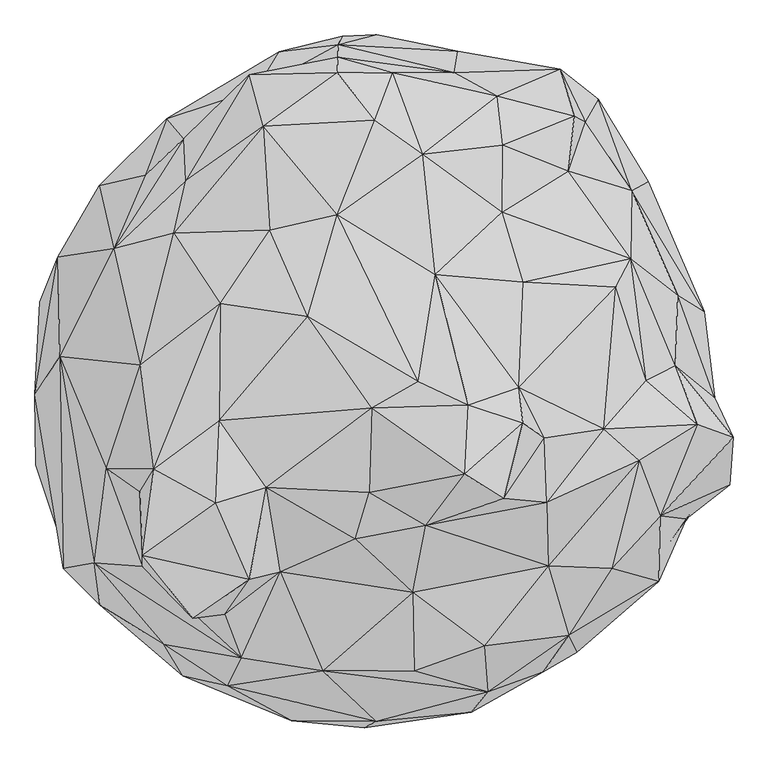
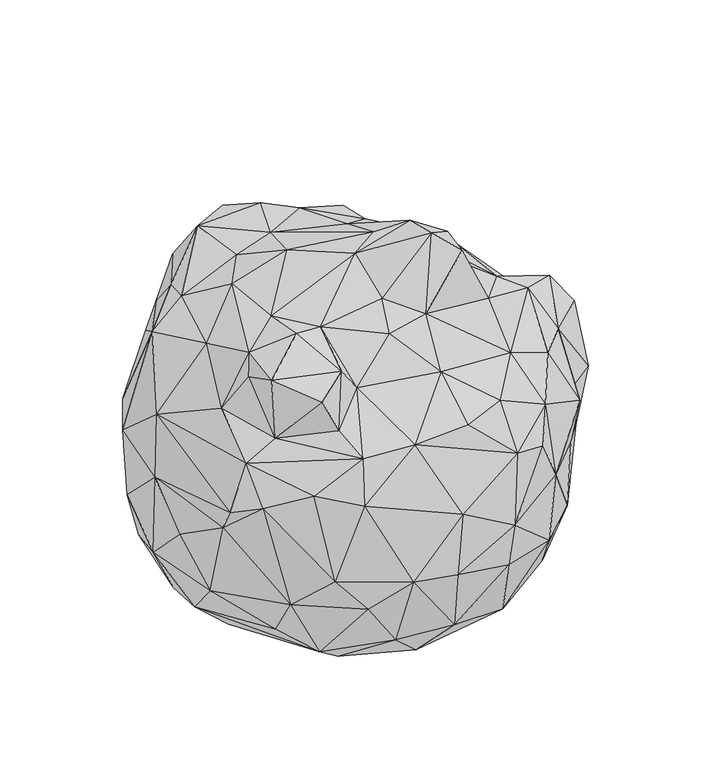
"""IFC4 building model written with IfcOpenShell, lengths in millimetres: geographic element geometry, Enscape AssetDefinition - Bush 001 Balm Bush : Enscape AssetDefinition - Bush 001 Balm Bush."""

from ifc_helpers import new_model, si_unit, origin, place, context, project, spatial, faceted_brep, source, transform, mapped, element, save


def geographic_element_0c4992a3(model_context):
    return source(origin(), model_context, "Body", "Brep", [
        faceted_brep([(-103.2708213, -28.0293748, 87.4930173), (344.7891772, -278.2743871, 87.4930173), (121.6873899, -550.0509143, 87.4930173), (312.7504289, -485.3526056, 87.4930173), (537.6026034, -111.360997, 122.5993857), (31.9034122, 85.9397277, 106.1995625), (483.1260741, 50.9389266, 117.1098575), (301.1055291, 161.4273489, 145.9610015), (-443.3142543, -218.7629938, 87.4930173), (-317.2000349, 6.4054755, 115.6498641), (-249.1122484, 226.8746197, 170.0659692), (94.6265161, 492.8733408, 281.8422019), (390.8439279, 296.7088819, 194.9024647), (518.7944174, 159.3808234, 184.8918945), (213.8534337, 460.0220025, 271.2863088), (425.7422388, 371.6726303, 251.8079579), (571.9012618, 134.5211118, 239.2979264), (542.7101851, 313.1485879, 468.670696), (379.9126446, 478.785485, 348.4884501), (445.0309277, 472.5328982, 451.1599839), (204.6146989, 556.6639304, 384.8151863), (510.0300908, 295.0474024, 639.8970485), (420.6644893, 429.313153, 672.0098257), (371.8031645, 530.8707952, 587.9698992), (650.9532332, 60.9223247, 488.0606234), (599.1232991, 92.9313004, 678.4057021), (508.5837245, 163.8322026, 850.7678509), (387.6252174, 333.4215879, 830.0852776), (398.8237381, 439.2881989, 790.2318835), (258.9309216, 253.3104122, 980.7052612), (260.5757713, 383.2080066, 949.7843385), (249.8932481, 478.099972, 884.2920661), (105.5608988, 366.3907349, 1005.6074858), (299.9075055, 118.1322485, 1021.5417147), (129.529193, 131.8538785, 1082.4985504), (47.3745875, 524.1814256, 883.228898), (12.6913656, 432.1153164, 1015.0117874), (-60.5219491, 248.3438998, 1047.7212667), (165.8966839, 524.0991116, 726.0334492), (-60.8999804, 523.4262943, 976.347208), (-59.549503, 553.7672043, 822.6758242), (-203.7955672, 420.4857647, 1017.4963474), (-230.6382805, 519.813776, 867.0647144), (-58.2677908, 578.6400437, 560.2571964), (-217.2929198, 491.6258454, 723.5295773), (173.101142, 566.0328269, 493.6592281), (15.6866908, 597.2068906, 333.124131), (-172.4721193, 564.8728609, 497.937113), (-50.7058874, 595.2501297, 355.7927608), (-390.5587792, 435.1478517, 548.4309793), (-357.5637639, 396.4434266, 820.2494979), (-343.9708948, 442.8346157, 317.6766038), (-372.1790016, 377.2239387, 247.8975356), (-237.534374, 397.4771798, 235.202238), (-479.7798395, 40.6567864, 115.3686419), (-473.3586311, 183.7875992, 165.3854996), (-502.1672845, 310.5277717, 338.2746279), (-566.3319826, 135.0266039, 225.5846113), (-637.4351978, 79.2079121, 425.8950949), (-601.8330455, 166.0981923, 590.0059342), (-521.4918852, 305.3177297, 587.0153904), (-540.3149724, -20.7758527, 124.5407835), (-645.5538869, -87.3326957, 326.2942135), (-485.3806496, -245.1593429, 111.8686944), (-579.3501139, -210.9759301, 185.881868), (-644.705832, -236.6477698, 479.1609049), (-646.4878321, -100.2570987, 598.8438129), (-594.2829251, -327.2557259, 317.9192841), (-464.2079473, -479.5174897, 227.9132307), (-352.8320491, -542.8832173, 148.7132013), (-455.3643167, -551.6501665, 355.2601039), (-271.4672089, -680.8964014, 353.6209464), (-170.5118865, -666.5790081, 202.0171285), (-285.6132984, -532.9383612, 102.6492417), (-591.2223458, -396.5682685, 580.4986358), (-521.1909413, -507.8048706, 690.6690598), (-591.9779539, -437.338084, 658.8361859), (-359.9068522, -645.4859972, 459.941864), (-148.5068798, -733.5099578, 437.9141033), (-396.7211545, -585.1808786, 738.4177446), (-273.3705044, -665.6394005, 709.523201), (-531.3819647, -427.161932, 807.2852492), (-598.5030532, -26.1186399, 759.1011524), (-508.1710815, -243.2810217, 880.5730343), (-438.2089078, -433.5936904, 865.5333519), (-246.6039956, -610.5666757, 833.7258697), (-88.9153406, -636.6765499, 844.8604345), (-170.9100604, -443.9971745, 956.7247629), (-278.5761952, -526.8044472, 893.348515), (15.429561, -733.9650393, 620.2399731), (231.3562334, -676.6399145, 726.3646126), (86.1066207, -484.4261408, 947.5157857), (88.954322, -636.2065077, 852.5073528), (224.4531512, -587.3548985, 861.1423969), (348.3548462, -432.8074157, 891.8932676), (111.0403612, -353.9148867, 1065.9604073), (-25.0923093, -380.2599907, 1058.245182), (387.8862858, -567.8147078, 777.7100205), (345.3665376, -310.0345433, 1011.2187862), (524.972558, -228.3504009, 935.6176853), (471.6629982, -437.2110367, 852.3084521), (339.2041624, -637.9516721, 691.8114424), (403.8853049, -599.8657942, 542.9646969), (562.8346205, -462.8386199, 667.9671407), (565.5180812, -335.6069624, 842.4683213), (543.7597036, -445.9197521, 519.1505551), (616.3422465, -341.9879079, 634.5546842), (636.9858384, -158.2563668, 898.1446028), (700.1382709, -275.8756578, 628.4427047), (706.8634629, -183.504194, 800.0890613), (632.6106191, -320.7831979, 469.7009921), (496.0250258, -506.0352087, 345.8895385), (597.0824957, -272.9684114, 188.5565519), (694.5405006, -162.4348462, 503.6548376), (666.3972139, -232.2055995, 314.5858049), (671.0886359, -106.4899862, 513.7941837), (594.8883295, -44.487454, 771.445632), (646.2192535, -58.1617877, 356.3556671), (511.9303465, -329.6220005, 145.768255), (406.0667455, -518.4435844, 190.7577068), (220.6544578, -612.2706532, 142.0440227), (380.6358278, -603.4296751, 321.4735389), (184.3929738, -707.8516483, 366.9776917), (11.4893802, -691.2187934, 205.8644295), (-75.4184127, -621.0311055, 106.2972471), (-157.6553881, -553.2301664, 87.4930173), (-7.666158, -746.5350628, 423.5813916), (199.0914494, -717.0593143, 507.3672533), (538.1067991, -72.7551207, 873.780787), (479.3207943, 108.591713, 904.4874907), (455.8838308, -167.5695628, 964.8863077), (291.7309999, -86.5770802, 1084.6892595), (340.4398561, -184.2843294, 1059.3217611), (193.4082955, -120.8397746, 1224.5627642), (298.9223301, -155.5948406, 1171.4243889), (261.9477212, -301.9075692, 1205.515027), (186.9322956, -254.3039024, 1264.8140192), (96.8473852, -75.4188523, 1191.7635202), (6.1829505, -126.3385117, 1176.9108772), (-117.9513335, 51.0777831, 1126.2102127), (-197.9201138, -280.4838419, 1082.4097395), (1.5169365, -289.9889052, 1118.8482046), (-289.5162702, -150.8416384, 1075.7974386), (-296.0483432, -310.9500408, 1113.3135557), (-231.2011719, -458.6890638, 1046.2844372), (-287.4570489, 75.9326741, 1049.9675274), (-416.0194695, -244.8229343, 1048.0645895), (-438.0349815, -411.9614661, 1058.3431721), (-340.1862383, -534.9345207, 1020.7331181), (-443.3633387, -289.6481156, 998.6404777), (-442.3177242, -43.1812182, 965.6659961), (-493.9005673, 182.8322262, 887.7061009), (-377.6369989, 212.3513818, 956.7554593), (-432.6637387, 325.3379762, 786.0648036), (-353.9012969, 314.6484196, 926.5795946), (-191.2693381, 219.0464139, 1032.8195095)], [[[0, 1, 2]], [[3, 1, 4]], [[5, 1, 0]], [[3, 2, 1]], [[1, 6, 4]], [[7, 6, 1]], [[1, 5, 7]], [[8, 9, 0]], [[8, 0, 2]], [[5, 0, 9]], [[10, 7, 5]], [[9, 10, 5]], [[10, 11, 7]], [[12, 7, 11]], [[12, 6, 7]], [[6, 12, 13]], [[6, 13, 4]], [[14, 15, 12]], [[12, 15, 13]], [[14, 12, 11]], [[15, 16, 13]], [[13, 16, 4]], [[15, 17, 16]], [[18, 15, 14]], [[15, 18, 19]], [[17, 15, 19]], [[11, 20, 14]], [[14, 20, 18]], [[18, 20, 19]], [[21, 17, 19]], [[22, 19, 23]], [[19, 22, 21]], [[20, 23, 19]], [[21, 24, 17]], [[16, 17, 24]], [[21, 25, 24]], [[26, 21, 27]], [[25, 21, 26]], [[27, 21, 22]], [[23, 28, 22]], [[22, 28, 27]], [[29, 27, 30]], [[27, 29, 26]], [[30, 27, 28]], [[31, 30, 28]], [[31, 28, 23]], [[32, 30, 31]], [[32, 29, 30]], [[29, 33, 26]], [[33, 29, 34]], [[34, 29, 32]], [[35, 32, 31]], [[35, 36, 32]], [[32, 36, 37]], [[32, 37, 34]], [[38, 35, 31]], [[31, 23, 38]], [[39, 35, 40]], [[39, 36, 35]], [[38, 40, 35]], [[36, 41, 37]], [[41, 36, 39]], [[42, 39, 40]], [[41, 39, 42]], [[43, 40, 38]], [[40, 43, 44]], [[40, 44, 42]], [[45, 38, 23]], [[38, 45, 43]], [[45, 23, 20]], [[43, 45, 46]], [[46, 45, 20]], [[43, 47, 44]], [[48, 47, 43]], [[46, 48, 43]], [[47, 49, 44]], [[50, 42, 44]], [[49, 50, 44]], [[48, 51, 47]], [[47, 51, 49]], [[51, 48, 52]], [[52, 48, 53]], [[46, 53, 48]], [[46, 11, 53]], [[20, 11, 46]], [[11, 10, 53]], [[53, 54, 55]], [[52, 53, 55]], [[53, 10, 54]], [[51, 52, 56]], [[57, 56, 52]], [[57, 52, 55]], [[51, 56, 49]], [[56, 58, 59]], [[57, 58, 56]], [[56, 60, 49]], [[60, 56, 59]], [[61, 57, 55]], [[57, 62, 58]], [[61, 62, 57]], [[54, 61, 55]], [[61, 63, 64]], [[64, 62, 61]], [[61, 54, 8]], [[61, 8, 63]], [[62, 65, 66]], [[62, 66, 58]], [[64, 67, 62]], [[62, 67, 65]], [[67, 64, 68]], [[68, 64, 69]], [[64, 63, 69]], [[63, 8, 69]], [[69, 70, 68]], [[71, 70, 69]], [[72, 71, 69]], [[69, 73, 72]], [[69, 8, 73]], [[68, 70, 67]], [[67, 70, 74]], [[67, 74, 65]], [[74, 66, 65]], [[74, 70, 75]], [[74, 76, 66]], [[75, 76, 74]], [[75, 70, 77]], [[70, 71, 77]], [[71, 78, 77]], [[72, 78, 71]], [[79, 77, 80]], [[78, 80, 77]], [[79, 75, 77]], [[79, 81, 75]], [[76, 75, 81]], [[66, 76, 82]], [[81, 82, 76]], [[83, 81, 84]], [[81, 85, 84]], [[81, 83, 82]], [[81, 79, 85]], [[79, 80, 85]], [[86, 87, 85]], [[80, 86, 85]], [[84, 85, 88]], [[85, 87, 88]], [[86, 89, 90]], [[91, 87, 86]], [[86, 92, 91]], [[80, 89, 86]], [[92, 86, 90]], [[91, 92, 93]], [[93, 92, 90]], [[94, 91, 93]], [[91, 94, 95]], [[96, 87, 91]], [[96, 91, 95]], [[93, 97, 94]], [[97, 93, 90]], [[94, 98, 95]], [[99, 98, 94]], [[94, 97, 100]], [[100, 99, 94]], [[97, 101, 102]], [[90, 101, 97]], [[102, 103, 97]], [[97, 103, 100]], [[104, 99, 100]], [[103, 104, 100]], [[105, 103, 102]], [[103, 105, 106]], [[103, 106, 104]], [[107, 99, 104]], [[108, 104, 106]], [[104, 108, 109]], [[104, 109, 107]], [[106, 105, 110]], [[108, 106, 110]], [[111, 110, 105]], [[105, 102, 111]], [[111, 112, 110]], [[113, 108, 110]], [[114, 113, 110]], [[110, 112, 114]], [[113, 109, 108]], [[115, 116, 109]], [[107, 109, 116]], [[109, 113, 115]], [[117, 113, 114]], [[117, 115, 113]], [[117, 114, 16]], [[114, 112, 4]], [[16, 114, 4]], [[118, 4, 112]], [[111, 118, 112]], [[118, 3, 4]], [[119, 118, 111]], [[3, 118, 119]], [[120, 3, 119]], [[2, 3, 120]], [[119, 121, 120]], [[111, 121, 119]], [[122, 123, 120]], [[124, 2, 120]], [[121, 122, 120]], [[123, 124, 120]], [[125, 2, 124]], [[125, 8, 2]], [[73, 125, 124]], [[72, 124, 123]], [[72, 73, 124]], [[125, 73, 8]], [[54, 9, 8]], [[10, 9, 54]], [[72, 123, 78]], [[123, 126, 78]], [[80, 78, 89]], [[89, 78, 126]], [[123, 122, 126]], [[122, 127, 126]], [[127, 89, 126]], [[90, 89, 127]], [[102, 127, 121]], [[101, 127, 102]], [[90, 127, 101]], [[121, 127, 122]], [[121, 111, 102]], [[117, 16, 24]], [[25, 115, 24]], [[115, 117, 24]], [[115, 25, 116]], [[116, 25, 26]], [[26, 128, 116]], [[128, 107, 116]], [[128, 26, 129]], [[26, 33, 129]], [[128, 130, 107]], [[129, 130, 128]], [[130, 99, 107]], [[130, 131, 132]], [[131, 130, 129]], [[132, 98, 130]], [[130, 98, 99]], [[33, 131, 129]], [[34, 131, 33]], [[34, 133, 131]], [[134, 132, 131]], [[133, 134, 131]], [[98, 132, 135]], [[134, 135, 132]], [[95, 98, 135]], [[135, 136, 95]], [[135, 134, 136]], [[136, 134, 133]], [[133, 34, 137]], [[138, 133, 137]], [[138, 136, 133]], [[37, 137, 34]], [[139, 138, 137]], [[137, 37, 139]], [[140, 141, 138]], [[141, 136, 138]], [[138, 139, 142]], [[138, 142, 140]], [[136, 141, 95]], [[141, 96, 95]], [[141, 140, 96]], [[140, 142, 143]], [[140, 87, 96]], [[144, 87, 140]], [[144, 140, 143]], [[145, 146, 142]], [[145, 142, 139]], [[142, 146, 143]], [[143, 147, 144]], [[143, 146, 147]], [[87, 144, 88]], [[88, 144, 148]], [[144, 147, 148]], [[84, 148, 147]], [[149, 84, 147]], [[147, 146, 149]], [[84, 88, 148]], [[84, 149, 83]], [[149, 146, 83]], [[145, 150, 146]], [[146, 150, 83]], [[83, 150, 82]], [[151, 82, 150]], [[145, 152, 150]], [[150, 152, 151]], [[59, 82, 151]], [[66, 82, 59]], [[59, 151, 60]], [[66, 59, 58]], [[153, 49, 60]], [[151, 153, 60]], [[49, 153, 50]], [[151, 50, 153]], [[50, 154, 42]], [[151, 154, 50]], [[154, 152, 41]], [[154, 41, 42]], [[152, 154, 151]], [[155, 41, 152]], [[37, 41, 155]], [[139, 37, 155]], [[139, 155, 145]], [[155, 152, 145]]]),
    ])


if __name__ == "__main__":
    model = new_model("IFC4")
    model_context = context("Model", 3, world=origin())
    ifc_project = project(units=[si_unit("LENGTHUNIT", "METRE", prefix="MILLI")], contexts=[model_context])
    site = spatial("IfcSite", under=ifc_project)
    building = spatial("IfcBuilding", under=site)
    placement = place(None, origin())
    geographic_element_shape = geographic_element_0c4992a3(model_context)
    element("IfcGeographicElement", 1, ObjectType="Enscape AssetDefinition - Bush 001 Balm Bush : Enscape AssetDefinition - Bush 001 Balm Bush", at=placement, inside=building, context=model_context, shape_type="MappedRepresentation", body=[
        mapped(geographic_element_shape, transform((0.0, 0.0, 0.0), x_axis=(1.0, 0.0, 0.0), y_axis=(0.0, 1.0, 0.0), z_axis=(0.0, 0.0, 1.0))),
    ])
    save(model, "model.ifc")

# Revit data of these elements
# Type "Enscape AssetDefinition - Bush 001 Balm Bush : Enscape AssetDefinition - Bush 001 Balm Bush"
#   EnscapeAssetSource = "REMOTE"
#   EnscapeAssetId = "42c5d65b-22f5-46ce-91d1-55bcf3f2a2d0"
#   Height = 1.264814 m
#   EnscapeNativeAssetHeight = 1.264814 m
#   Default Elevation = 0
